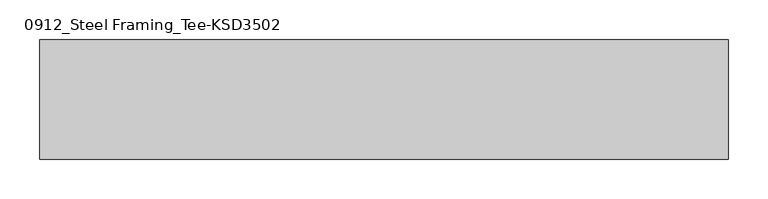
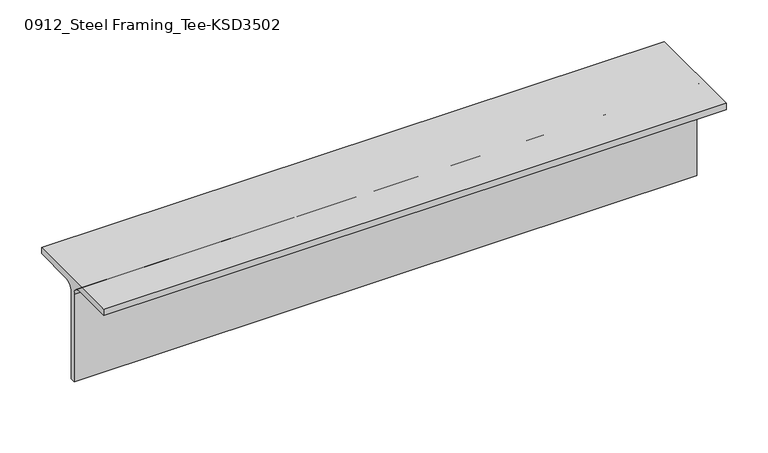
"""IFC4 building model written with IfcOpenShell, lengths in millimetres: member geometry, 0912_Steel Framing_Tee-KSD3502 : H_SB_ASB_CT-150x150x6.5x9."""

from ifc_helpers import new_model, si_unit, point, frame, frame_2d, origin, place, context, project, spatial, polyline, circle_curve, trimmed, segment, composite_curve, outline, extrude, source, transform, mapped, element, save


def member_0912_steel_framing_tee_ksd3502_749f5b2d(model_context):
    return source(origin(), model_context, "Body", "SweptSolid", [
        extrude(outline(composite_curve([segment(polyline([(75.0, 75.0), (75.0, 66.0), (16.25, 66.0)]), True, "CONTINUOUS"), segment(trimmed(circle_curve(frame_2d((16.25, 53.0)), 13.0), [point((16.25, 66.0))], [point((3.25, 53.0))], True, "CARTESIAN"), True, "CONTINUOUS"), segment(polyline([(3.25, 53.0), (3.25, -75.0), (-3.25, -75.0), (-3.25, 53.0)]), True, "CONTINUOUS"), segment(trimmed(circle_curve(frame_2d((-16.25, 53.0)), 13.0), [point((-3.25, 53.0))], [point((-16.25, 66.0))], True, "CARTESIAN"), True, "CONTINUOUS"), segment(polyline([(-16.25, 66.0), (-75.0, 66.0), (-75.0, 75.0), (75.0, 75.0)]), True, "CONTINUOUS")], self_intersect=False)), frame((-500.0, 0.0, 0.0), z_axis=(1.0, 0.0, 0.0), x_axis=(0.0, 1.0, 0.0)), (0.0, 0.0, 1.0), 865.9),
    ])


if __name__ == "__main__":
    model = new_model("IFC4")
    model_context = context("Model", 3, world=origin())
    ifc_project = project(units=[si_unit("LENGTHUNIT", "METRE", prefix="MILLI")], contexts=[model_context])
    site = spatial("IfcSite", under=ifc_project)
    building = spatial("IfcBuilding", under=site)
    placement = place(None, origin())
    member_0912_steel_framing_tee_ksd3502_shape = member_0912_steel_framing_tee_ksd3502_749f5b2d(model_context)
    element("IfcMember", 1, ObjectType="0912_Steel Framing_Tee-KSD3502 : H_SB_ASB_CT-150x150x6.5x9", at=placement, inside=building, context=model_context, shape_type="MappedRepresentation", body=[
        mapped(member_0912_steel_framing_tee_ksd3502_shape, transform((0.0, 0.0, 0.0), x_axis=(1.0, 0.0, 0.0), y_axis=(0.0, 1.0, 0.0), z_axis=(0.0, 0.0, 1.0))),
    ])
    save(model, "model.ifc")

# Revit data of these elements
# Type "0912_Steel Framing_Tee-KSD3502 : H_SB_ASB_CT-150x150x6.5x9"
#   H_WM Code_1 = "S01AA003-00001 | Main Steel Structure Fabrication Work | Shelter/Building | Light Steel - Standard (30KG/M>Weight) | Material: (   )"
#   H_WM Code_2 = "S03AA029-00001 | Main Steel Structure Erection Work | Shelter/Building | Light Steel (30KG/M>Weight) | Material: (   )"
#   H_WM Code_3 = "S01AA010-00001 | Main Steel Structure Fabrication Work | Shelter/Building | Steel Painting/Coating | for Non-Fireproofed Steel Surface, Surface Preparation, Primer, Second & Final Coat | Material: (   )"
#   H_Q'ty Cal Type Tag = "SB-Q2"
#   Width = 15.0 cm
#   Web Thickness = 0.65 cm
#   Web Fillet = 1.3 cm
#   Section Area = 23.39 cm²
#   Perimeter = 0.60 m²/m
#   Nominal Weight = 18.40 kgf/m
#   Height = 15.0 cm
#   Flange Thickness = 0.9 cm
#   Centroid Vertical = 7.5 cm
#   Centroid Horizontal = 7.5 cm
#   Length [instance default] = 1.5000 m
#   Structural Material [instance default] = Steel, 45-345
#   Warping Constant = (empty or 0)
#   Torsional Moment of Inertia = 0
#   Section Name Key = ""
#   Plastic Modulus weak axis = 0
#   Plastic Modulus strong axis = 0
#   Moment of Inertia weak axis = 0
#   Moment of Inertia strong axis = 0
#   Elastic Modulus weak axis = 0
#   Elastic Modulus strong axis = 0
#   Bolt Spacing = 0
#   Assembly Code = ""
# Element 1 (IfcMember, "0912_Steel Framing_Tee-KSD3502 : H_SB_ASB_CT-150x150x6.5x9")
#   Structural Material = none
# Materials
#   "Steel, 45-345": class "Metal", colour RGB 189 187 185, transparency 0, Description = "Steel 345 MPa", Cost = 0
